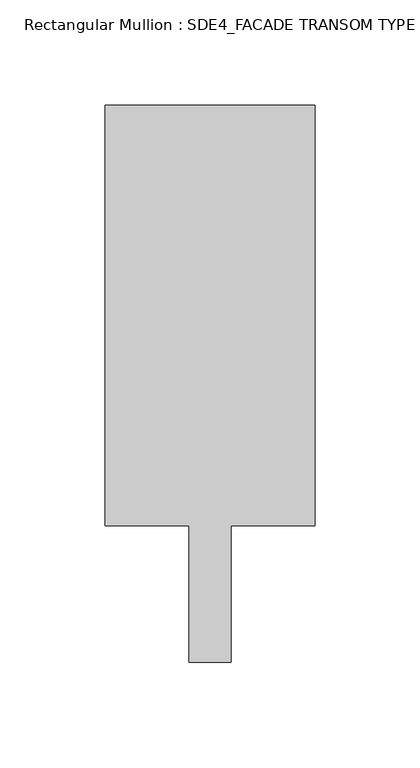
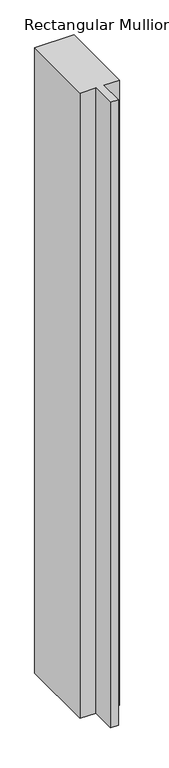
"""IFC4 building model written with IfcOpenShell, lengths in millimetres: member geometry, Rectangular Mullion : SDE4_FACADE TRANSOM TYPE 2."""

from ifc_helpers import new_model, si_unit, frame, origin, place, context, project, spatial, polyline, outline, extrude, source, transform, mapped, element, save


def rectangular_mullion_sde4_facade_transom_type_2_288c81da(model_context):
    return source(origin(), model_context, "Body", "SweptSolid", [
        extrude(outline(polyline([(50.0, 132.5), (50.0, -67.5), (10.0, -67.5), (10.0, -132.5), (-10.0, -132.5), (-10.0, -67.5), (-50.0, -67.5), (-50.0, 132.5), (50.0, 132.5)])), frame((0.0, 0.0, -1681.5), z_axis=(0.0, 0.0, 1.0), x_axis=(1.0, 0.0, 0.0)), (0.0, 0.0, 1.0), 1681.5),
    ])


if __name__ == "__main__":
    model = new_model("IFC4")
    model_context = context("Model", 3, world=origin())
    ifc_project = project(units=[si_unit("LENGTHUNIT", "METRE", prefix="MILLI")], contexts=[model_context])
    site = spatial("IfcSite", under=ifc_project)
    building = spatial("IfcBuilding", under=site)
    placement = place(None, origin())
    rectangular_mullion_sde4_facade_transom_type_2_shape = rectangular_mullion_sde4_facade_transom_type_2_288c81da(model_context)
    element("IfcMember", 1, ObjectType="Rectangular Mullion : SDE4_FACADE TRANSOM TYPE 2", at=placement, inside=building, context=model_context, shape_type="MappedRepresentation", body=[
        mapped(rectangular_mullion_sde4_facade_transom_type_2_shape, transform((0.0, 0.0, 0.0), x_axis=(1.0, 0.0, 0.0), y_axis=(0.0, 1.0, 0.0), z_axis=(0.0, 0.0, 1.0))),
    ])
    save(model, "model.ifc")

# Revit data of these elements
# Type "Rectangular Mullion : SDE4_FACADE TRANSOM TYPE 2"
#   built-in parameter 1007322 = 0.869423 (stored number, unit not read)
#   built-in parameter 1007321 = 0.164042 (stored number, unit not read)
#   built-in parameter 1007320 = 0.164042 (stored number, unit not read)
